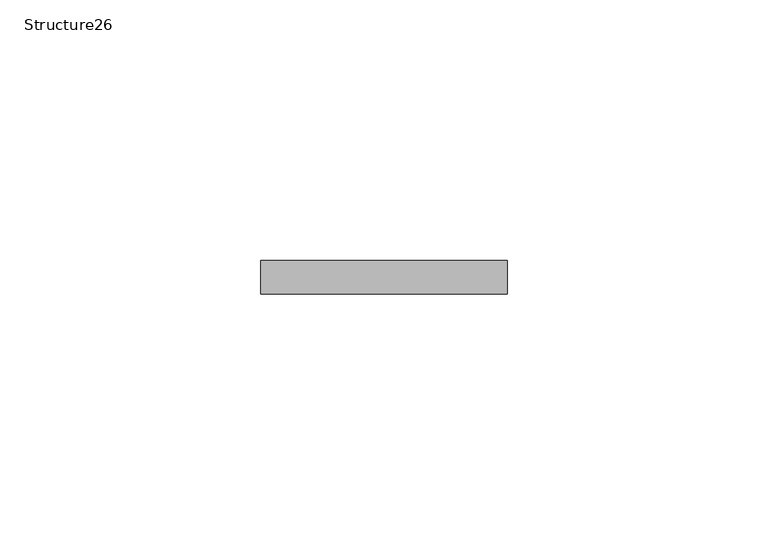
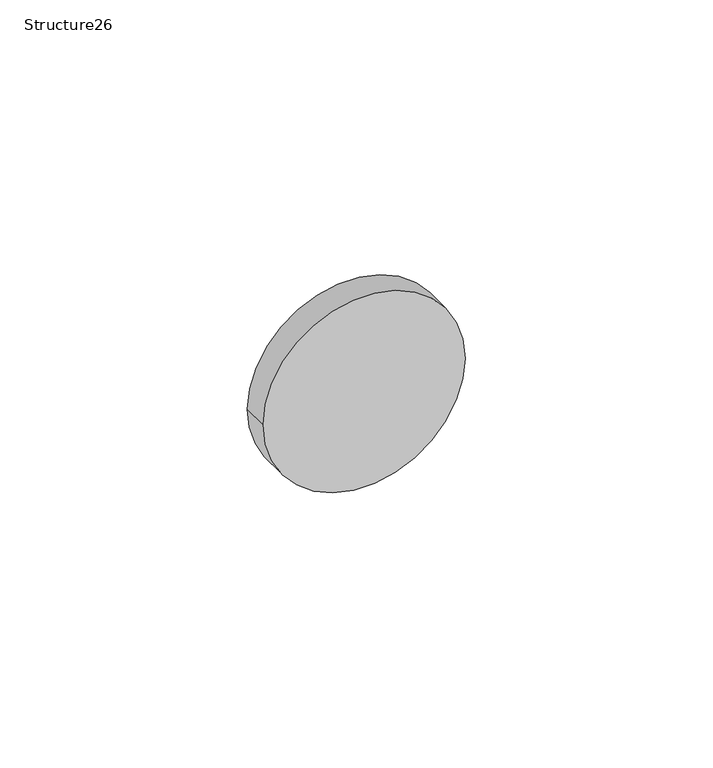
"""IFC4 building model written with IfcOpenShell, lengths in millimetres: proxy geometry, Structure26 : Structure668217154."""

from ifc_helpers import new_model, si_unit, point, frame, frame_2d, origin, place, context, project, spatial, circle_curve, trimmed, segment, composite_curve, outline, extrude, source, transform, mapped, element, save


def structure26_dcf3c21a(model_context):
    return source(origin(), model_context, "Body", "SweptSolid", [
        extrude(outline(composite_curve([segment(trimmed(circle_curve(frame_2d((40908.7088339, 9847.8795269)), 23.5716554), [point((40908.7088339, 9824.3078714))], [point((40908.7088339, 9871.4511823))], False, "CARTESIAN"), True, "CONTINUOUS"), segment(trimmed(circle_curve(frame_2d((40908.7088339, 9847.8795269)), 23.5716554), [point((40908.7088339, 9871.4511823))], [point((40908.7088339, 9824.3078714))], False, "CARTESIAN"), True, "CONTINUOUS")], self_intersect=False)), frame((0.0, 1926.1573723, 0.0), z_axis=(0.0, 1.0, 0.0), x_axis=(0.0, 0.0, 1.0)), (0.0, 0.0, 1.0), 6.35),
    ])


if __name__ == "__main__":
    model = new_model("IFC4")
    model_context = context("Model", 3, world=origin())
    ifc_project = project(units=[si_unit("LENGTHUNIT", "METRE", prefix="MILLI")], contexts=[model_context])
    site = spatial("IfcSite", under=ifc_project)
    building = spatial("IfcBuilding", under=site)
    placement = place(None, origin())
    structure26_shape = structure26_dcf3c21a(model_context)
    element("IfcBuildingElementProxy", 1, Name="Structure26 : Structure668217154", ObjectType="Structure26 : Structure668217154", at=placement, inside=building, context=model_context, shape_type="MappedRepresentation", body=[
        mapped(structure26_shape, transform((0.0, 0.0, 0.0), x_axis=(1.0, 0.0, 0.0), y_axis=(0.0, 1.0, 0.0), z_axis=(0.0, 0.0, 1.0))),
    ])
    save(model, "model.ifc")

# Revit data of these elements
# Type "Structure26 : Structure668217154"
#   NameOverride = "Structure668217154"
# Element 1 (IfcBuildingElementProxy, "Structure26 : Structure668217154")
#   Materials on its faces: "RUBBER GASKET"
# Materials
#   "RUBBER GASKET": class "Unassigned", colour RGB 70 70 70, transparency 0
